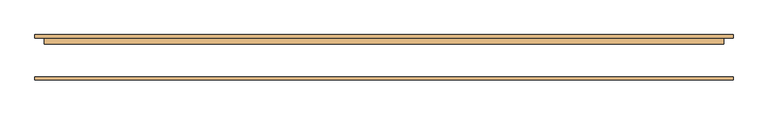
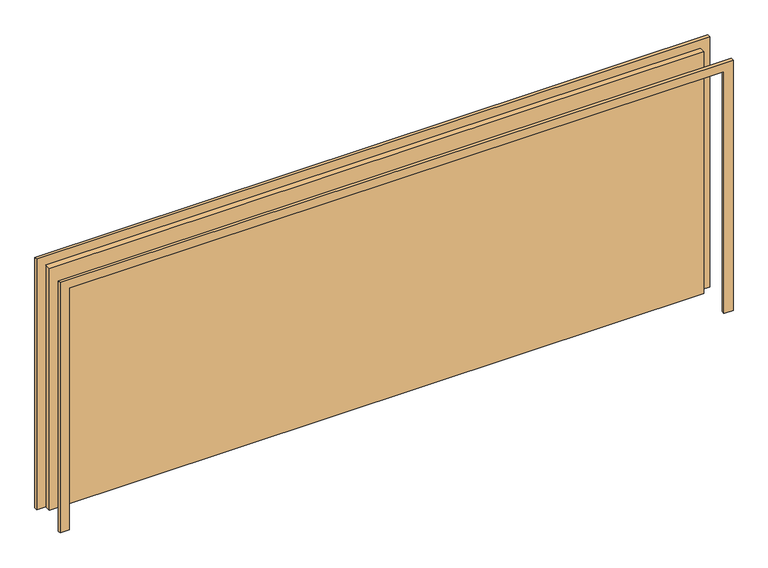
"""IFC4 building model written with IfcOpenShell, lengths in millimetres: door geometry."""

from ifc_helpers import new_model, si_unit, frame, origin, origin_with_axes, place, context, project, spatial, polyline, outline, extrude, source, transform, mapped, element, save


def door_79ccea0e(model_context):
    return source(origin(), model_context, "Body", "SweptSolid", [
        extrude(outline(polyline([(2209.8, -2806.7), (0.0, -2806.7), (0.0, -2730.5), (2133.6, -2730.5), (2133.6, 2730.5), (0.0, 2730.5), (0.0, 2806.7), (2209.8, 2806.7), (2209.8, -2806.7)])), frame((0.0, 157.1625, 0.0), z_axis=(0.0, 1.0, 0.0), x_axis=(0.0, 0.0, 1.0)), (0.0, 0.0, 1.0), 25.4),
        extrude(outline(polyline([(2209.8, 2806.7), (2209.8, -2806.7), (0.0, -2806.7), (0.0, -2730.5), (2133.6, -2730.5), (2133.6, 2730.5), (0.0, 2730.5), (0.0, 2806.7), (2209.8, 2806.7)])), frame((0.0, -182.5625, 0.0), z_axis=(0.0, 1.0, 0.0), x_axis=(0.0, 0.0, 1.0)), (0.0, 0.0, 1.0), 25.4),
        extrude(outline(polyline([(2730.5, 106.3625), (-2730.5, 106.3625), (-2730.5, 157.1625), (2730.5, 157.1625), (2730.5, 106.3625)])), origin_with_axes(), (0.0, 0.0, 1.0), 2133.6),
    ])


if __name__ == "__main__":
    model = new_model("IFC4")
    model_context = context("Model", 3, world=origin())
    ifc_project = project(units=[si_unit("LENGTHUNIT", "METRE", prefix="MILLI")], contexts=[model_context])
    site = spatial("IfcSite", under=ifc_project)
    building = spatial("IfcBuilding", under=site)
    placement = place(None, origin())
    door_shape = door_79ccea0e(model_context)
    element("IfcDoor", 1, ObjectType="project specific garage door : 215\" x 84\"-Garrage", at=placement, inside=building, context=model_context, shape_type="MappedRepresentation", body=[
        mapped(door_shape, transform((0.0, 0.0, 0.0), x_axis=(1.0, 0.0, 0.0), y_axis=(0.0, 1.0, 0.0), z_axis=(0.0, 0.0, 1.0))),
    ])
    save(model, "model.ifc")

# Revit data of these elements
# Type "project specific garage door : 215\" x 84\"-Garrage"
#   Type Mark = "23"
#   Construction Type Id = "MDOOR"
#   Assembly Code = "C1020"
#   Analytic Construction = "Metal"
#   Thickness = 0' - 2"
#   Thermal Resistance (R) = 0.270117 (m²·K)/W
#   Heat Transfer Coefficient (U) = 3.7021 W/(m²·K)
#   Height = 7' - 0"
#   Trim Projection Ext = 0' - 1"
#   Trim Projection Int = 0' - 1"
#   Trim Width = 0' - 3"
#   Width = 17' - 11"
#   Door Material = Metal Trim
#   Frame Material = Metal Trim
#   Visual Light Transmittance = 0
#   Solar Heat Gain Coefficient = 0
#   Function = (empty or 0)
#   Wall Closure = (empty or 0)
# Element 1 (IfcDoor, "project specific garage door : 215\" x 84\"-Garrage")
#   Materials on its faces: "Metal Trim"
# Materials
#   "Metal Trim": class "Wood", colour RGB 151 137 121, transparency 0, Cost = 0
